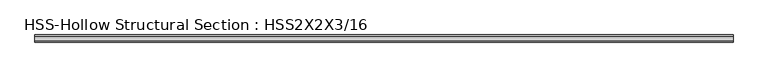
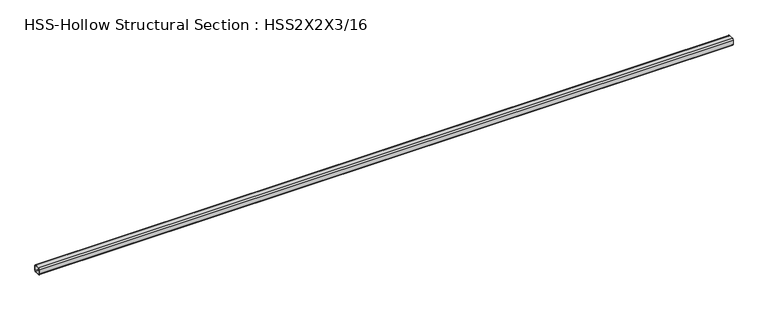
"""IFC4 building model written with IfcOpenShell, lengths in millimetres: beam geometry, HSS-Hollow Structural Section : HSS2X2X3/16."""

from ifc_helpers import new_model, si_unit, point, frame, frame_2d, origin, place, context, project, spatial, polyline, circle_curve, trimmed, segment, composite_curve, outline, extrude, source, transform, mapped, element, save


def hss_hollow_structural_section_hss2x2x3_16_1b2ea3b5(model_context):
    return source(origin(), model_context, "Body", "SweptSolid", [
        extrude(outline(composite_curve([segment(polyline([(25.4, 16.5608), (25.4, -16.5608)]), True, "CONTINUOUS"), segment(trimmed(circle_curve(frame_2d((16.5608, -16.5608)), 8.8392), [point((25.4, -16.5608))], [point((16.5608, -25.4))], False, "CARTESIAN"), True, "CONTINUOUS"), segment(polyline([(16.5608, -25.4), (-16.5608, -25.4)]), True, "CONTINUOUS"), segment(trimmed(circle_curve(frame_2d((-16.5608, -16.5608)), 8.8392), [point((-16.5608, -25.4))], [point((-25.4, -16.5608))], False, "CARTESIAN"), True, "CONTINUOUS"), segment(polyline([(-25.4, -16.5608), (-25.4, 16.5608)]), True, "CONTINUOUS"), segment(trimmed(circle_curve(frame_2d((-16.5608, 16.5608)), 8.8392), [point((-25.4, 16.5608))], [point((-16.5608, 25.4))], False, "CARTESIAN"), True, "CONTINUOUS"), segment(polyline([(-16.5608, 25.4), (16.5608, 25.4)]), True, "CONTINUOUS"), segment(trimmed(circle_curve(frame_2d((16.5608, 16.5608)), 8.8392), [point((16.5608, 25.4))], [point((25.4, 16.5608))], False, "CARTESIAN"), True, "CONTINUOUS")], self_intersect=False), holes=[composite_curve([segment(trimmed(circle_curve(frame_2d((-16.5608, 16.5608)), 4.4196), [point((-16.5608, 20.9804))], [point((-20.9804, 16.5608))], True, "CARTESIAN"), True, "CONTINUOUS"), segment(polyline([(-20.9804, 16.5608), (-20.9804, -16.5608)]), True, "CONTINUOUS"), segment(trimmed(circle_curve(frame_2d((-16.5608, -16.5608)), 4.4196), [point((-20.9804, -16.5608))], [point((-16.5608, -20.9804))], True, "CARTESIAN"), True, "CONTINUOUS"), segment(polyline([(-16.5608, -20.9804), (16.5608, -20.9804)]), True, "CONTINUOUS"), segment(trimmed(circle_curve(frame_2d((16.5608, -16.5608)), 4.4196), [point((16.5608, -20.9804))], [point((20.9804, -16.5608))], True, "CARTESIAN"), True, "CONTINUOUS"), segment(polyline([(20.9804, -16.5608), (20.9804, 16.5608)]), True, "CONTINUOUS"), segment(trimmed(circle_curve(frame_2d((16.5608, 16.5608)), 4.4196), [point((20.9804, 16.5608))], [point((16.5608, 20.9804))], True, "CARTESIAN"), True, "CONTINUOUS"), segment(polyline([(16.5608, 20.9804), (-16.5608, 20.9804)]), True, "CONTINUOUS")], self_intersect=False)]), frame((4545.80625, 0.0, 0.0), z_axis=(1.0, 0.0, 0.0), x_axis=(0.0, 1.0, 0.0)), (0.0, 0.0, 1.0), 4943.475),
    ])


if __name__ == "__main__":
    model = new_model("IFC4")
    model_context = context("Model", 3, world=origin())
    ifc_project = project(units=[si_unit("LENGTHUNIT", "METRE", prefix="MILLI")], contexts=[model_context])
    site = spatial("IfcSite", under=ifc_project)
    building = spatial("IfcBuilding", under=site)
    placement = place(None, origin())
    hss_hollow_structural_section_hss2x2x3_16_shape = hss_hollow_structural_section_hss2x2x3_16_1b2ea3b5(model_context)
    element("IfcBeam", 1, ObjectType="HSS-Hollow Structural Section : HSS2X2X3/16", at=placement, inside=building, context=model_context, shape_type="MappedRepresentation", body=[
        mapped(hss_hollow_structural_section_hss2x2x3_16_shape, transform((0.0, 0.0, 0.0), x_axis=(1.0, 0.0, 0.0), y_axis=(0.0, 1.0, 0.0), z_axis=(0.0, 0.0, 1.0))),
    ])
    save(model, "model.ifc")

# Revit data of these elements
# Type "HSS-Hollow Structural Section : HSS2X2X3/16"
#   Keynote = "M05121300.04"
#   Assembly Code = "B10"
#   Shape = "Square"
#   W = 4.3
#   Ht = 0' - 2"
#   Length [instance default] = 5' - 0"
#   b = 0' - 2"
#   kr = 0' - 0.348"
#   t = 0' - 0.174"
#   A = 0.00826389 SF
#   Structural Material [instance default] = Steel ASTM A500, Grade B, Rectangular and Square
# Element 1 (IfcBeam, "HSS-Hollow Structural Section : HSS2X2X3/16")
#   Materials on its faces: "Steel ASTM A500, Grade B, Rectangular and Square"
# Materials
#   "Steel ASTM A500, Grade B, Rectangular and Square": class "Metal", colour RGB 199 199 199, transparency 0, Description = "Carbon steel", Cost = 0
